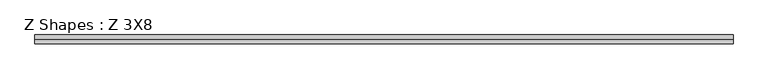
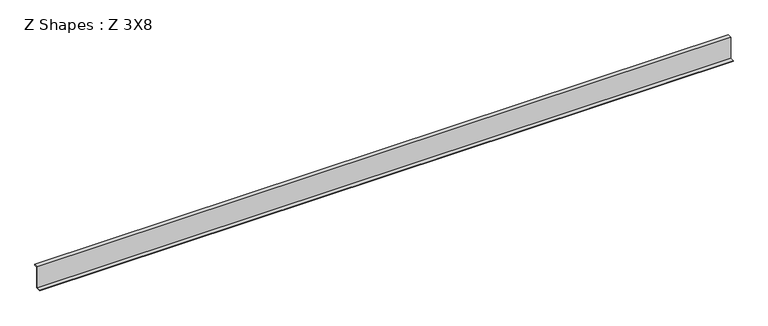
"""IFC4 building model written with IfcOpenShell, lengths in millimetres: beam geometry, Z Shapes : Z 3X8."""

from ifc_helpers import new_model, si_unit, frame, origin, place, context, project, spatial, polyline, outline, extrude, source, transform, mapped, element, save


def z_shapes_z_3x8_41227fe0(model_context):
    return source(origin(), model_context, "Body", "SweptSolid", [
        extrude(outline(polyline([(57.2805719, 92.452825), (27.1991352, 92.452825), (27.1991352, -98.809175), (-18.9194281, -98.809175), (-18.9194281, -92.459175), (19.1805719, -92.459175), (19.1805719, 102.104825), (57.2805719, 102.104825), (57.2805719, 92.452825)])), frame((-11474.45, 0.0, 0.0), z_axis=(1.0, 0.0, 0.0), x_axis=(0.0, 1.0, 0.0)), (0.0, 0.0, 1.0), 6108.7),
    ])


if __name__ == "__main__":
    model = new_model("IFC4")
    model_context = context("Model", 3, world=origin())
    ifc_project = project(units=[si_unit("LENGTHUNIT", "METRE", prefix="MILLI")], contexts=[model_context])
    site = spatial("IfcSite", under=ifc_project)
    building = spatial("IfcBuilding", under=site)
    placement = place(None, origin())
    z_shapes_z_3x8_shape = z_shapes_z_3x8_41227fe0(model_context)
    element("IfcBeam", 1, ObjectType="Z Shapes : Z 3X8", at=placement, inside=building, context=model_context, shape_type="MappedRepresentation", body=[
        mapped(z_shapes_z_3x8_shape, transform((0.0, 0.0, 0.0), x_axis=(1.0, 0.0, 0.0), y_axis=(0.0, 1.0, 0.0), z_axis=(0.0, 0.0, 1.0))),
    ])
    save(model, "model.ifc")

# Revit data of these elements
# Type "Z Shapes : Z 3X8"
#   Section Name Key = "W12x26"
#   Assembly Code = "B10"
#   Width = 76.2 mm
#   Web Thickness = 5.842 mm
#   Web Fillet = 7.62 mm
#   Warping Constant = 163001.3 cm⁶
#   Torsional Moment of Inertia = 12.4869 cm⁴
#   Section Area = 7.65 in²
#   Plastic Modulus weak axis = 0.00472801 (stored number, unit not read)
#   Plastic Modulus strong axis = 0.0215278 (stored number, unit not read)
#   Perimeter = 15.0571 m²/m
#   Nominal Weight = 379.441 N/m
#   Moment of Inertia weak axis = 720.08 cm⁴
#   Moment of Inertia strong axis = 8491.12 cm⁴
#   Height = 184.912 mm
#   Flange Thickness = 9.652 mm
#   Elastic Modulus weak axis = 0.00309028 (stored number, unit not read)
#   Elastic Modulus strong axis = 0.0193287 (stored number, unit not read)
#   Centroid Vertical = 92.456 mm
#   Centroid Horizontal = 38.1 mm
#   Length [instance default] = 5' - 0"
#   Structural Material [instance default] = Steel ASTM A992
#   Principal Axes Angle = 0
# Element 1 (IfcBeam, "Z Shapes : Z 3X8")
#   Materials on its faces: "Steel ASTM A992"
# Materials
#   "Steel ASTM A992": class "Metal", colour RGB 189 187 185, transparency 0, Description = "Structural steel 50ksi", Cost = 0
